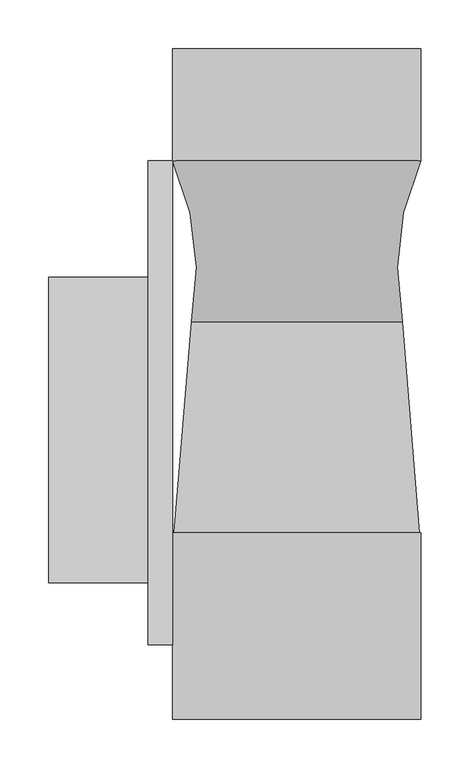
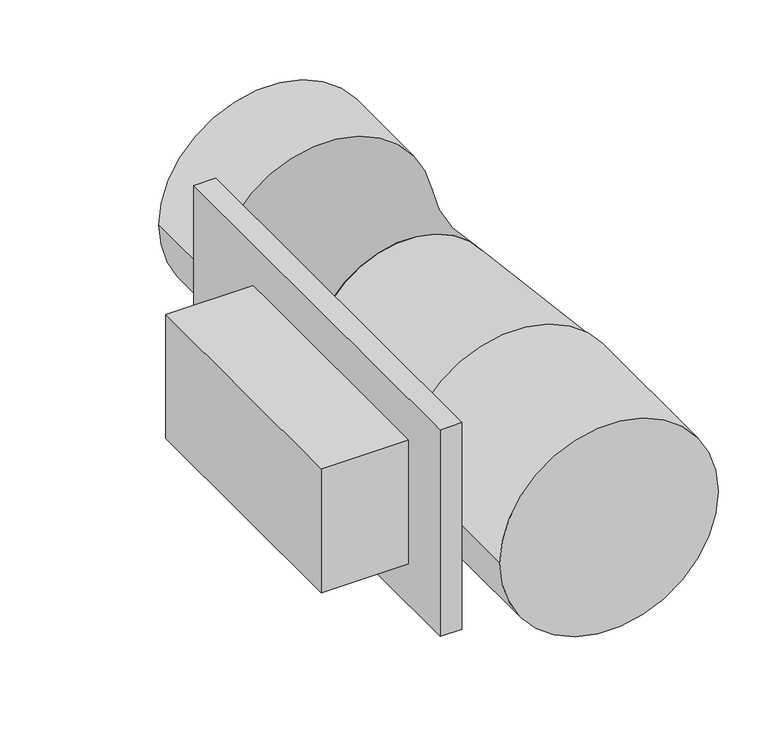
"""IFC4 building model written with IfcOpenShell, lengths in millimetres: proxy geometry, PValve250 : PValve250."""

from ifc_helpers import new_model, si_unit, point, frame, origin, origin_2d, place, context, project, spatial, polyline, circle_curve, ellipse_curve, trimmed, segment, composite_curve, outline, extrude, source, transform, mapped, element, save
from ifc_brep_helpers import plane_surface, revolved_surface, advanced_brep


def mechanical_equipment_f1c23132(model_context):
    return source(origin(), model_context, "Body", "SolidModel", [
        advanced_brep(
        [(127.0, -114.3, 0.0), (-127.0, -114.3, 0.0), (-101.6, -114.3, 0.0), (101.6, -114.3, 0.0), (-107.95, -279.4, 0.0), (107.95, -279.4, 0.0), (101.6, -279.4, 0.0), (-101.6, -279.4, 0.0)],
        [
            (0, 1, circle_curve(frame((0.0, -114.3, 0.0), z_axis=(0.0, 1.0, 0.0), x_axis=(1.0, 0.0, 0.0)), 127.0)),
            (1, 2),
            (2, 3, circle_curve(frame((0.0, -114.3, 0.0), z_axis=(0.0, -1.0, 0.0), x_axis=(1.0, 0.0, 0.0)), 101.6)),
            (3, 0),
            (1, 0, circle_curve(frame((0.0, -114.3, 0.0), z_axis=(0.0, 1.0, 0.0), x_axis=(1.0, 0.0, 0.0)), 127.0)),
            (3, 2, circle_curve(frame((0.0, -114.3, 0.0), z_axis=(0.0, -1.0, 0.0), x_axis=(1.0, 0.0, 0.0)), 101.6)),
            (4, 5, circle_curve(frame((0.0, -279.4, 0.0), z_axis=(0.0, -1.0, 0.0), x_axis=(1.0, 0.0, 0.0)), 107.95)),
            (5, 6),
            (6, 7, circle_curve(frame((0.0, -279.4, 0.0), z_axis=(0.0, 1.0, 0.0), x_axis=(1.0, 0.0, 0.0)), 101.6)),
            (7, 4),
            (5, 4, circle_curve(frame((0.0, -279.4, 0.0), z_axis=(0.0, -1.0, 0.0), x_axis=(1.0, 0.0, 0.0)), 107.95)),
            (7, 6, circle_curve(frame((0.0, -279.4, 0.0), z_axis=(0.0, 1.0, 0.0), x_axis=(1.0, 0.0, 0.0)), 101.6)),
            (6, 3),
            (2, 7),
            (0, 5, circle_curve(frame((375.8082613, -226.657684, 0.0), z_axis=(0.0, 0.0, 1.0), x_axis=(1.0, 0.0, 0.0)), 273.0014653)),
            (4, 1, circle_curve(frame((-375.8082613, -226.657684, 0.0), z_axis=(0.0, 0.0, 1.0), x_axis=(-1.0, 0.0, 0.0)), 273.0014653)),
        ],
        [
            plane_surface(frame((0.0, -114.3, 0.0), z_axis=(0.0, 1.0, 0.0), x_axis=(1.0, 0.0, 0.0))),
            plane_surface(frame((0.0, -279.4, 0.0), z_axis=(0.0, -1.0, 0.0), x_axis=(1.0, 0.0, 0.0))),
            revolved_surface(polyline([(101.6, -279.4, 0.0), (101.6, -114.3, 0.0)]), (0.0, 0.0, 0.0), (0.0, -1.0, 0.0)),
            revolved_surface(trimmed(ellipse_curve(frame((375.8082613, -226.657684, 0.0), z_axis=(0.0, 0.0, -1.0), x_axis=(1.0, 0.0, 0.0)), 273.0014653, 273.0014653), [point((107.95, -279.4, 0.0))], [point((127.0, -114.3, 0.0))], True, "CARTESIAN"), (0.0, -114.3, 0.0), (0.0, 1.0, 0.0)),
        ],
        [
            (0, [[1, 2, 3, 4]]),
            (0, [[5, -4, 6, -2]]),
            (1, [[7, 8, 9, 10]]),
            (1, [[11, -10, 12, -8]]),
            (2, [[13, -3, 14, -9]]),
            (2, [[-13, -12, -14, -6]]),
            (3, [[-1, 15, -7, 16]]),
            (3, [[-5, -16, -11, -15]]),
        ],
    ),
        extrude(outline(composite_curve([segment(trimmed(circle_curve(origin_2d(), 127.0), [point((0.0, -127.0))], [point((0.0, 127.0))], False, "CARTESIAN"), True, "CONTINUOUS"), segment(trimmed(circle_curve(origin_2d(), 127.0), [point((0.0, 127.0))], [point((0.0, -127.0))], False, "CARTESIAN"), True, "CONTINUOUS")], self_intersect=False), holes=[composite_curve([segment(trimmed(circle_curve(origin_2d(), 101.6), [point((0.0, 101.6))], [point((0.0, -101.6))], True, "CARTESIAN"), True, "CONTINUOUS"), segment(trimmed(circle_curve(origin_2d(), 101.6), [point((0.0, -101.6))], [point((0.0, 101.6))], True, "CARTESIAN"), True, "CONTINUOUS")], self_intersect=False)]), frame((0.0, -114.3, 0.0), z_axis=(0.0, 1.0, 0.0), x_axis=(0.0, 0.0, 1.0)), (0.0, 0.0, 1.0), 114.3),
        extrude(outline(polyline([(-254.0, -546.1), (-254.0, -233.5601781), (-152.4, -233.5601781), (-152.4, -546.1), (-254.0, -546.1)])), frame((0.0, 0.0, -76.2), z_axis=(0.0, 0.0, 1.0), x_axis=(1.0, 0.0, 0.0)), (0.0, 0.0, 1.0), 152.4),
        extrude(outline(polyline([(-127.0, -609.6), (-152.4, -609.6), (-152.4, -114.3), (-127.0, -114.3), (-127.0, -609.6)])), frame((0.0, 0.0, -127.0), z_axis=(0.0, 0.0, 1.0), x_axis=(1.0, 0.0, 0.0)), (0.0, 0.0, 1.0), 254.0),
        extrude(outline(composite_curve([segment(trimmed(circle_curve(origin_2d(), 127.0), [point((0.0, -127.0))], [point((0.0, 127.0))], False, "CARTESIAN"), True, "CONTINUOUS"), segment(trimmed(circle_curve(origin_2d(), 127.0), [point((0.0, 127.0))], [point((0.0, -127.0))], False, "CARTESIAN"), True, "CONTINUOUS")], self_intersect=False)), frame((0.0, -685.8, 0.0), z_axis=(0.0, 1.0, 0.0), x_axis=(0.0, 0.0, 1.0)), (0.0, 0.0, 1.0), 190.5),
        advanced_brep(
        [(0.0, -495.3, 0.0), (-125.6148395, -495.3, 0.0), (125.6148395, -495.3, 0.0), (107.95, -279.4, 0.0), (-107.95, -279.4, 0.0), (0.0, -279.4, 0.0)],
        [
            (0, 1),
            (1, 2, circle_curve(frame((0.0, -495.3, 0.0), z_axis=(0.0, -1.0, 0.0), x_axis=(-1.0, 0.0, 0.0)), 125.6148395)),
            (2, 0),
            (2, 1, circle_curve(frame((0.0, -495.3, 0.0), z_axis=(0.0, -1.0, 0.0), x_axis=(-1.0, 0.0, 0.0)), 125.6148395)),
            (3, 4, circle_curve(frame((0.0, -279.4, 0.0), z_axis=(0.0, 1.0, 0.0), x_axis=(-1.0, 0.0, 0.0)), 107.95)),
            (4, 5),
            (5, 3),
            (4, 3, circle_curve(frame((0.0, -279.4, 0.0), z_axis=(0.0, 1.0, 0.0), x_axis=(-1.0, 0.0, 0.0)), 107.95)),
            (1, 4),
            (3, 2),
        ],
        [
            plane_surface(frame((0.0, -495.3, 0.0), z_axis=(0.0, -1.0, 0.0), x_axis=(-1.0, 0.0, 0.0))),
            plane_surface(frame((0.0, -279.4, 0.0), z_axis=(0.0, 1.0, 0.0), x_axis=(-1.0, 0.0, 0.0))),
            revolved_surface(polyline([(-107.95, -279.4, 0.0), (-125.6148395, -495.3, 0.0)]), (0.0, -279.4, 0.0), (0.0, -1.0, 0.0)),
        ],
        [
            (0, [[1, 2, 3]]),
            (0, [[-3, 4, -1]]),
            (1, [[5, 6, 7]]),
            (1, [[8, -7, -6]]),
            (2, [[-2, 9, -5, 10]]),
            (2, [[-4, -10, -8, -9]]),
        ],
    ),
    ])


if __name__ == "__main__":
    model = new_model("IFC4")
    model_context = context("Model", 3, world=origin())
    ifc_project = project(units=[si_unit("LENGTHUNIT", "METRE", prefix="MILLI")], contexts=[model_context])
    site = spatial("IfcSite", under=ifc_project)
    building = spatial("IfcBuilding", under=site)
    placement = place(None, origin())
    mechanical_equipment_shape = mechanical_equipment_f1c23132(model_context)
    element("IfcBuildingElementProxy", 1, Name="PValve250 : PValve250", ObjectType="PValve250 : PValve250", at=placement, inside=building, context=model_context, shape_type="MappedRepresentation", body=[
        mapped(mechanical_equipment_shape, transform((0.0, 0.0, 0.0), x_axis=(1.0, 0.0, 0.0), y_axis=(0.0, 1.0, 0.0), z_axis=(0.0, 0.0, 1.0))),
    ])
    save(model, "model.ifc")

# Revit data of these elements
# Type "PValve250 : PValve250"
#   Assembly Code = ""
